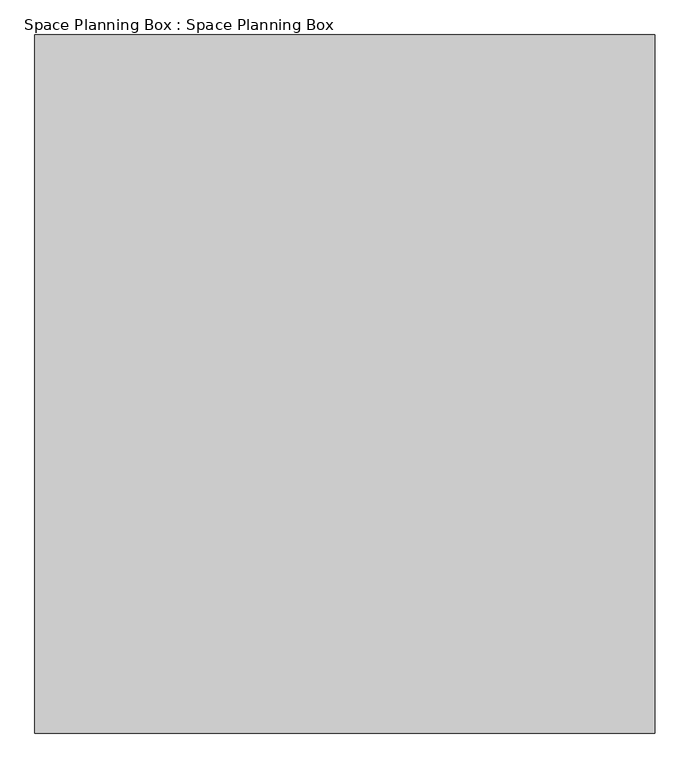
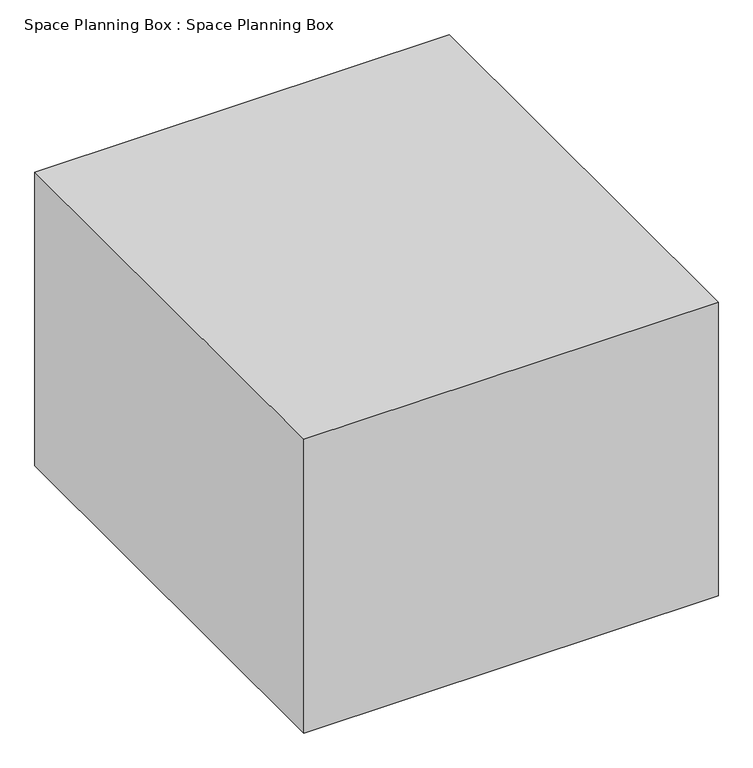
"""IFC4 building model written with IfcOpenShell, lengths in millimetres: proxy geometry, Space Planning Box : Space Planning Box."""

from ifc_helpers import new_model, si_unit, origin, origin_with_axes, place, context, project, spatial, polyline, outline, extrude, source, transform, mapped, element, save


def space_planning_box_space_planning_box_4d084078(model_context):
    return source(origin(), model_context, "Body", "SweptSolid", [
        extrude(outline(polyline([(4000.0, 4500.0), (4000.0, -4500.0), (-4000.0, -4500.0), (-4000.0, 4500.0), (4000.0, 4500.0)])), origin_with_axes(), (0.0, 0.0, 1.0), 6000.0),
    ])


if __name__ == "__main__":
    model = new_model("IFC4")
    model_context = context("Model", 3, world=origin())
    ifc_project = project(units=[si_unit("LENGTHUNIT", "METRE", prefix="MILLI")], contexts=[model_context])
    site = spatial("IfcSite", under=ifc_project)
    building = spatial("IfcBuilding", under=site)
    placement = place(None, origin())
    space_planning_box_space_planning_box_shape = space_planning_box_space_planning_box_4d084078(model_context)
    element("IfcBuildingElementProxy", 1, Name="Space Planning Box : Space Planning Box", ObjectType="Space Planning Box : Space Planning Box", at=placement, inside=building, context=model_context, shape_type="MappedRepresentation", body=[
        mapped(space_planning_box_space_planning_box_shape, transform((0.0, 0.0, 0.0), x_axis=(1.0, 0.0, 0.0), y_axis=(0.0, 1.0, 0.0), z_axis=(0.0, 0.0, 1.0))),
    ])
    save(model, "model.ifc")

# Revit data of these elements
# Type "Space Planning Box : Space Planning Box"
#   Type Comments = "..."
#   Room Name [instance default] = "?"
#   Assembly Code = "..."
#   Width [instance default] = 1524 mm
#   Program Area [instance default] = 0 m²
#   Length [instance default] = 1524 mm
#   Height [instance default] = 1524 mm
#   Area [instance default] = 2.32258 m²
#   Fill Color [instance default] = Cyan
#   Default Elevation = 0
# Element 1 (IfcBuildingElementProxy, "Space Planning Box : Space Planning Box")
#   Room Name = "Fire Gas Room"
#   Width = 8000 mm
#   Length = 9000 mm
#   Height = 6000 mm
#   Area = 72 m²
#   Materials on its faces: "Cyan"
# Materials
#   "Cyan": class "Generic", colour RGB 0 255 255, transparency 0.2, Cost = 0
